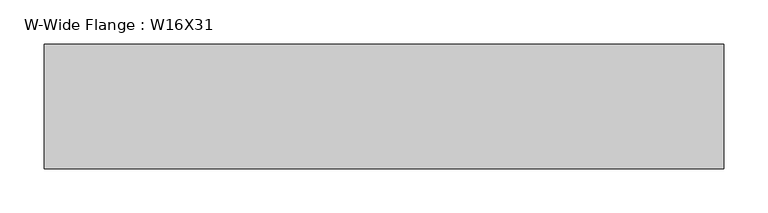
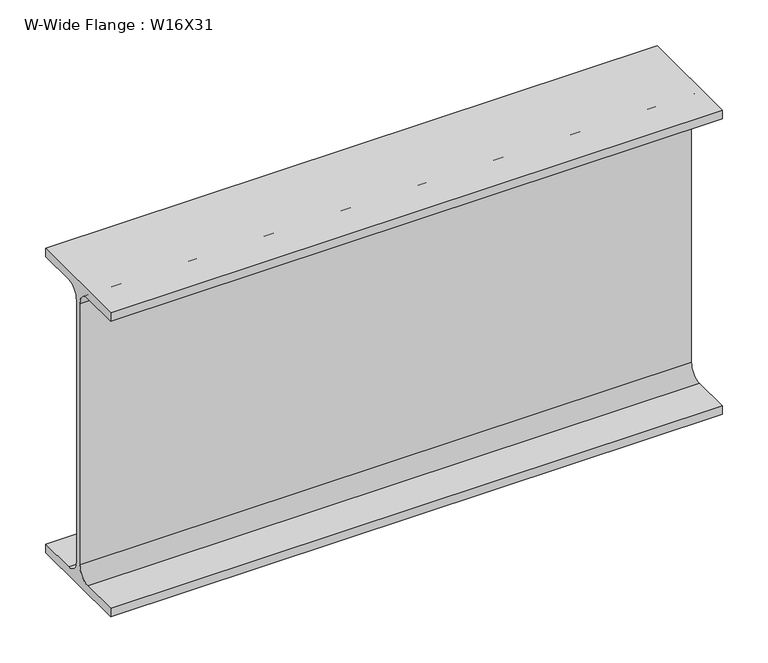
"""IFC4 building model written with IfcOpenShell, lengths in millimetres: beam geometry, W-Wide Flange : W16X31."""

from ifc_helpers import new_model, si_unit, point, frame, frame_2d, origin, place, context, project, spatial, polyline, circle_curve, trimmed, segment, composite_curve, outline, extrude, source, transform, mapped, element, save


def w_wide_flange_w16x31_03689333(model_context):
    return source(origin(), model_context, "Body", "SweptSolid", [
        extrude(outline(composite_curve([segment(polyline([(70.231, -190.754), (70.231, -201.93), (-70.231, -201.93), (-70.231, -190.754), (-20.8915, -190.754)]), True, "CONTINUOUS"), segment(trimmed(circle_curve(frame_2d((-20.8915, -173.355)), 17.399), [point((-20.8915, -190.754))], [point((-3.4925, -173.355))], True, "CARTESIAN"), True, "CONTINUOUS"), segment(polyline([(-3.4925, -173.355), (-3.4925, 173.355)]), True, "CONTINUOUS"), segment(trimmed(circle_curve(frame_2d((-20.8915, 173.355)), 17.399), [point((-3.4925, 173.355))], [point((-20.8915, 190.754))], True, "CARTESIAN"), True, "CONTINUOUS"), segment(polyline([(-20.8915, 190.754), (-70.231, 190.754), (-70.231, 201.93), (70.231, 201.93), (70.231, 190.754), (20.8915, 190.754)]), True, "CONTINUOUS"), segment(trimmed(circle_curve(frame_2d((20.8915, 173.355)), 17.399), [point((20.8915, 190.754))], [point((3.4925, 173.355))], True, "CARTESIAN"), True, "CONTINUOUS"), segment(polyline([(3.4925, 173.355), (3.4925, -173.355)]), True, "CONTINUOUS"), segment(trimmed(circle_curve(frame_2d((20.8915, -173.355)), 17.399), [point((3.4925, -173.355))], [point((20.8915, -190.754))], True, "CARTESIAN"), True, "CONTINUOUS"), segment(polyline([(20.8915, -190.754), (70.231, -190.754)]), True, "CONTINUOUS")], self_intersect=False)), frame((-355.5790981, 0.0, 0.0), z_axis=(1.0, 0.0, 0.0), x_axis=(0.0, 1.0, 0.0)), (0.0, 0.0, 1.0), 767.969),
    ])


if __name__ == "__main__":
    model = new_model("IFC4")
    model_context = context("Model", 3, world=origin())
    ifc_project = project(units=[si_unit("LENGTHUNIT", "METRE", prefix="MILLI")], contexts=[model_context])
    site = spatial("IfcSite", under=ifc_project)
    building = spatial("IfcBuilding", under=site)
    placement = place(None, origin())
    w_wide_flange_w16x31_shape = w_wide_flange_w16x31_03689333(model_context)
    element("IfcBeam", 1, ObjectType="W-Wide Flange : W16X31", at=placement, inside=building, context=model_context, shape_type="MappedRepresentation", body=[
        mapped(w_wide_flange_w16x31_shape, transform((0.0, 0.0, 0.0), x_axis=(1.0, 0.0, 0.0), y_axis=(0.0, 1.0, 0.0), z_axis=(0.0, 0.0, 1.0))),
    ])
    save(model, "model.ifc")

# Revit data of these elements
# Type "W-Wide Flange : W16X31"
#   Assembly Code = "B10"
#   W = 31
#   Start Extension Calculation [instance default] = 10' - 0"
#   Start Extension [instance default] = -0' - 0 1/2"
#   End Extension Calculation [instance default] = 10' - 0"
#   End Extension [instance default] = -0' - 0 1/2"
#   Length [instance default] = 5' - 0"
#   bf = 0' - 5.53"
#   d = 1' - 3.9"
#   k = 0' - 1 1/8"
#   k2 = 0' - 0.685"
#   tf = 0' - 0.44"
#   tw = 0' - 0.275"
#   A = 0.0634028 SF
#   Beam Material [instance default] = Metal - Steel - ASTM A992
# Element 1 (IfcBeam, "W-Wide Flange : W16X31")
#   Materials on its faces: "Metal - Steel - ASTM A992"
# Materials
#   "Metal - Steel - ASTM A992": class "Metal", colour RGB 128 0 0, transparency 0
